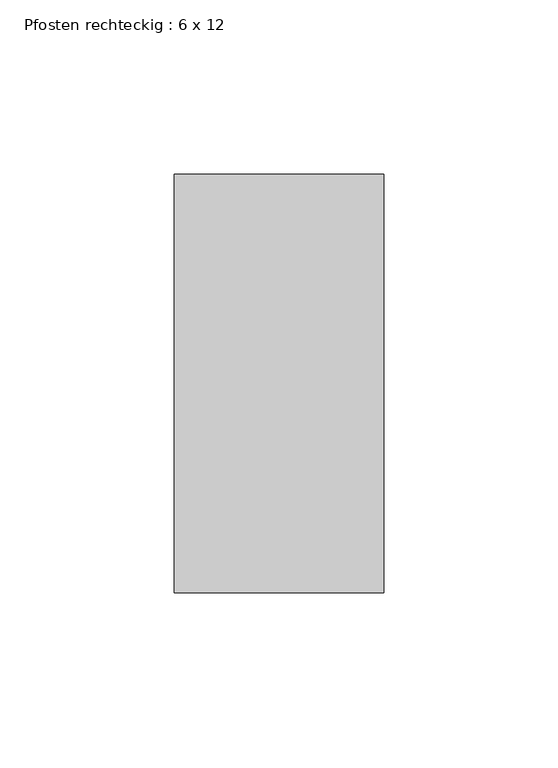
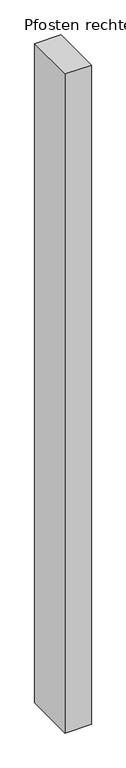
"""IFC4 building model written with IfcOpenShell, lengths in millimetres: member geometry, Pfosten rechteckig : 6 x 12."""

from ifc_helpers import new_model, si_unit, frame, origin, place, context, project, spatial, polyline, outline, extrude, source, transform, mapped, element, save


def pfosten_rechteckig_6_x_12_a5d0c5e5(model_context):
    return source(origin(), model_context, "Body", "SweptSolid", [
        extrude(outline(polyline([(0.0, 60.0), (0.0, -60.0), (-60.0, -60.0), (-60.0, 60.0), (0.0, 60.0)])), frame((0.0, 0.0, -1589.9495836), z_axis=(0.0, 0.0, 1.0), x_axis=(1.0, 0.0, 0.0)), (0.0, 0.0, 1.0), 1589.9495836),
    ])


if __name__ == "__main__":
    model = new_model("IFC4")
    model_context = context("Model", 3, world=origin())
    ifc_project = project(units=[si_unit("LENGTHUNIT", "METRE", prefix="MILLI")], contexts=[model_context])
    site = spatial("IfcSite", under=ifc_project)
    building = spatial("IfcBuilding", under=site)
    placement = place(None, origin())
    pfosten_rechteckig_6_x_12_shape = pfosten_rechteckig_6_x_12_a5d0c5e5(model_context)
    element("IfcMember", 1, ObjectType="Pfosten rechteckig : 6 x 12", at=placement, inside=building, context=model_context, shape_type="MappedRepresentation", body=[
        mapped(pfosten_rechteckig_6_x_12_shape, transform((0.0, 0.0, 0.0), x_axis=(1.0, 0.0, 0.0), y_axis=(0.0, 1.0, 0.0), z_axis=(0.0, 0.0, 1.0))),
    ])
    save(model, "model.ifc")

# Revit data of these elements
# Type "Pfosten rechteckig : 6 x 12"
#   built-in parameter 1007304 = 0.393701 (stored number, unit not read)
#   built-in parameter 1007301 = 0.0984252 (stored number, unit not read)
#   built-in parameter 1007300 = 0.0984252 (stored number, unit not read)
# Element 1 (IfcMember, "Pfosten rechteckig : 6 x 12")
#   Materials on its faces: "Metall - verzinkt"
# Materials
#   "Metall - verzinkt": class "Allgemeines", colour RGB 200 200 200, transparency 0, Cost = 0
